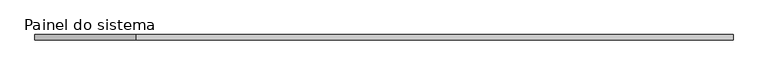
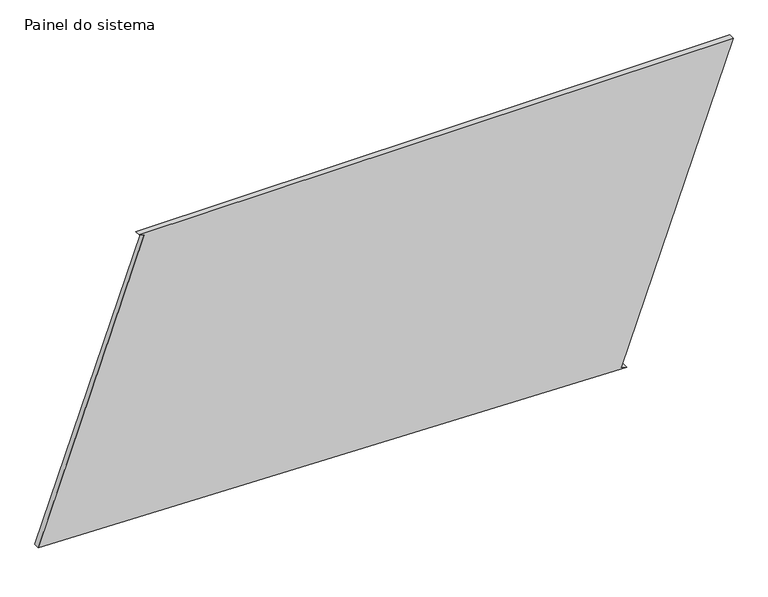
"""IFC4 building model written with IfcOpenShell, lengths in millimetres: plate geometry, Painel do sistema : Envidraçado."""

from ifc_helpers import new_model, si_unit, frame, origin, place, context, project, spatial, polyline, outline, extrude, source, transform, mapped, element, save


def painel_do_sistema_f27324c5(model_context):
    return source(origin(), model_context, "Body", "SweptSolid", [
        extrude(outline(polyline([(0.0, 1099.1628894), (8.505028, 1075.6540719), (1416.4493583, 1585.0206519), (1416.4493583, -1124.2063665), (1407.9443303, -1100.697549), (69.22288, -1585.0206519), (0.0, 1099.1628894)])), frame((0.0, 24.5, 0.0), z_axis=(0.0, 1.0, 0.0), x_axis=(0.0, 0.0, 1.0)), (0.0, 0.0, 1.0), 25.0),
    ])


if __name__ == "__main__":
    model = new_model("IFC4")
    model_context = context("Model", 3, world=origin())
    ifc_project = project(units=[si_unit("LENGTHUNIT", "METRE", prefix="MILLI")], contexts=[model_context])
    site = spatial("IfcSite", under=ifc_project)
    building = spatial("IfcBuilding", under=site)
    placement = place(None, origin())
    painel_do_sistema_shape = painel_do_sistema_f27324c5(model_context)
    element("IfcPlate", 1, ObjectType="Painel do sistema : Envidraçado", at=placement, inside=building, context=model_context, shape_type="MappedRepresentation", body=[
        mapped(painel_do_sistema_shape, transform((0.0, 0.0, 0.0), x_axis=(1.0, 0.0, 0.0), y_axis=(0.0, 1.0, 0.0), z_axis=(0.0, 0.0, 1.0))),
    ])
    save(model, "model.ifc")

# Revit data of these elements
# Type "Painel do sistema : Envidraçado"
#   Construction Type Id = "GSP4R"
#   Analytic Construction = "Vidraça única Pilkington 1/8 pol"
#   Visual Light Transmittance = 0.9
#   Solar Heat Gain Coefficient = 0.86
#   Heat Transfer Coefficient (U) = 6.7069 W/(m²·K)
# Element 1 (IfcPlate, "Painel do sistema : Envidraçado")
#   Materials on its faces: "Vidro"
# Materials
#   "Vidro": class "Vidro", colour RGB 0 128 192, transparency 0.9, Description = "Vidro de sílica", Cost = 0
